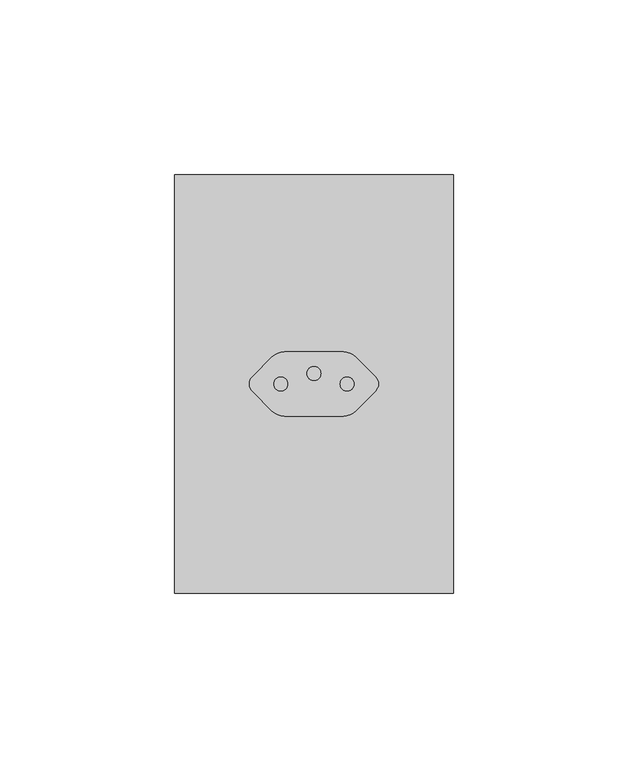
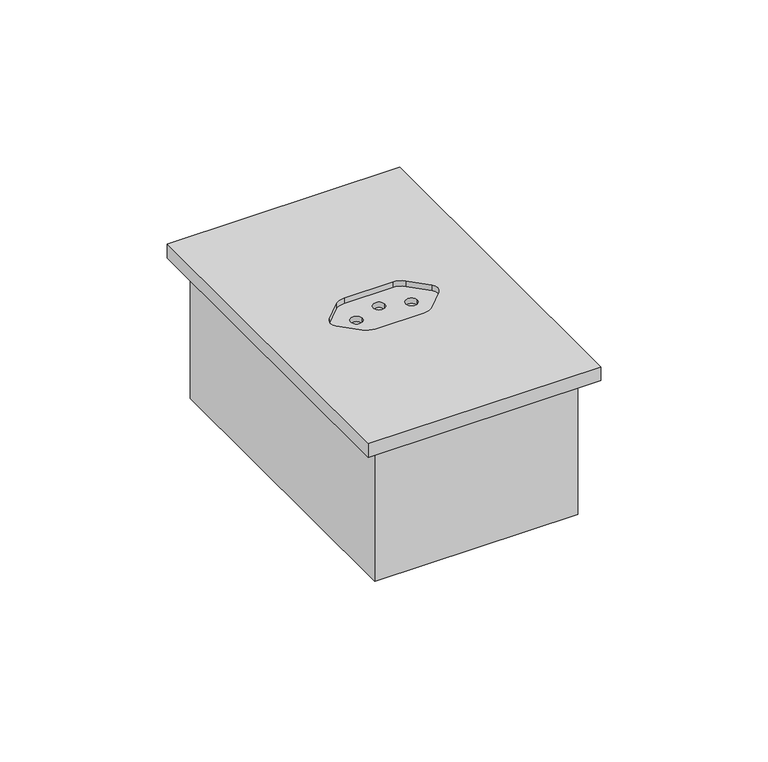
"""IFC4 building model written with IfcOpenShell, lengths in millimetres: proxy geometry, CAIXA VERTICE V7 : Tomada 10A 1s."""

from ifc_helpers import new_model, si_unit, frame, origin, place, context, project, spatial, polyline, circle_curve, faceted_brep, source, transform, mapped, element, save
from ifc_brep_helpers import plane_surface, revolved_surface, advanced_brep


def electrical_fixtures_2885af8d(model_context):
    return source(origin(), model_context, "Body", "SolidModel", [
        faceted_brep([(35.0, 455.0, 0.0), (-35.0, 455.0, 0.0), (-35.0, 345.0, 0.0), (35.0, 345.0, 0.0), (33.0, 453.0, 0.0), (33.0, 347.0, 0.0), (-33.0, 347.0, 0.0), (-33.0, 453.0, 0.0), (33.0, 347.0, -48.0), (33.0, 453.0, -48.0), (-33.0, 453.0, -48.0), (-33.0, 347.0, -48.0), (35.0, 455.0, -50.0), (35.0, 345.0, -50.0), (-35.0, 345.0, -50.0), (-35.0, 455.0, -50.0)], [[[0, 1, 2, 3], [4, 5, 6, 7]], [[8, 9, 10, 11]], [[12, 13, 14, 15]], [[12, 15, 1, 0]], [[1, 15, 14, 2]], [[2, 14, 13, 3]], [[3, 13, 12, 0]], [[5, 4, 9, 8]], [[6, 5, 8, 11]], [[7, 6, 11, 10]], [[4, 7, 10, 9]]]),
        advanced_brep(
        [(40.0, 460.0, 5.0), (-40.0, 460.0, 5.0), (-40.0, 340.0, 5.0), (40.0, 340.0, 5.0), (8.4215729, 390.75, 5.0), (-8.4215729, 390.75, 5.0), (-11.9571068, 392.2144661, 5.0), (-17.6213203, 397.8786797, 5.0), (-17.6213203, 402.1213203, 5.0), (-11.9571068, 407.7855339, 5.0), (-8.4215729, 409.25, 5.0), (8.4215729, 409.25, 5.0), (11.9571068, 407.7855339, 5.0), (17.6213203, 402.1213203, 5.0), (17.6213203, 397.8786797, 5.0), (11.9571068, 392.2144661, 5.0), (-40.0, 460.0, 0.0), (40.0, 460.0, 0.0), (40.0, 340.0, 0.0), (-40.0, 340.0, 0.0), (8.4215729, 390.75, 3.0), (11.9571068, 392.2144661, 3.0), (17.6213203, 397.8786797, 3.0), (17.6213203, 402.1213203, 3.0), (11.9571068, 407.7855339, 3.0), (8.4215729, 409.25, 3.0), (-8.4215729, 409.25, 3.0), (-11.9571068, 407.7855339, 3.0), (-17.6213203, 402.1213203, 3.0), (-17.6213203, 397.8786797, 3.0), (-11.9571068, 392.2144661, 3.0), (-8.4215729, 390.75, 3.0), (-7.5, 400.0, 3.0), (-11.5, 400.0, 3.0), (11.5, 400.0, 3.0), (7.5, 400.0, 3.0), (2.0, 403.0, 3.0), (-2.0, 403.0, 3.0), (-11.5, 400.0, 1.0), (-7.5, 400.0, 1.0), (7.5, 400.0, 1.0), (11.5, 400.0, 1.0), (-2.0, 403.0, 1.0), (2.0, 403.0, 1.0)],
        [
            (0, 1),
            (1, 2),
            (2, 3),
            (3, 0),
            (4, 5),
            (5, 6, circle_curve(frame((-8.4215729, 395.75, 5.0), z_axis=(0.0, 0.0, -1.0), x_axis=(-1.0, 0.0, 0.0)), 5.0)),
            (6, 7),
            (7, 8, circle_curve(frame((-15.5, 400.0, 5.0), z_axis=(0.0, 0.0, -1.0), x_axis=(-1.0, 0.0, 0.0)), 3.0)),
            (8, 9),
            (9, 10, circle_curve(frame((-8.4215729, 404.25, 5.0), z_axis=(0.0, 0.0, -1.0), x_axis=(-1.0, 0.0, 0.0)), 5.0)),
            (10, 11),
            (11, 12, circle_curve(frame((8.4215729, 404.25, 5.0), z_axis=(0.0, 0.0, -1.0), x_axis=(-1.0, 0.0, 0.0)), 5.0)),
            (12, 13),
            (13, 14, circle_curve(frame((15.5, 400.0, 5.0), z_axis=(0.0, 0.0, -1.0), x_axis=(-1.0, 0.0, 0.0)), 3.0)),
            (14, 15),
            (15, 4, circle_curve(frame((8.4215729, 395.75, 5.0), z_axis=(0.0, 0.0, -1.0), x_axis=(-1.0, 0.0, 0.0)), 5.0)),
            (16, 17),
            (17, 18),
            (18, 19),
            (19, 16),
            (0, 17),
            (16, 1),
            (19, 2),
            (18, 3),
            (20, 21, circle_curve(frame((8.4215729, 395.75, 3.0), z_axis=(0.0, 0.0, 1.0), x_axis=(-1.0, 0.0, 0.0)), 5.0)),
            (21, 22),
            (22, 23, circle_curve(frame((15.5, 400.0, 3.0), z_axis=(0.0, 0.0, 1.0), x_axis=(-1.0, 0.0, 0.0)), 3.0)),
            (23, 24),
            (24, 25, circle_curve(frame((8.4215729, 404.25, 3.0), z_axis=(0.0, 0.0, 1.0), x_axis=(-1.0, 0.0, 0.0)), 5.0)),
            (25, 26),
            (26, 27, circle_curve(frame((-8.4215729, 404.25, 3.0), z_axis=(0.0, 0.0, 1.0), x_axis=(-1.0, 0.0, 0.0)), 5.0)),
            (27, 28),
            (28, 29, circle_curve(frame((-15.5, 400.0, 3.0), z_axis=(0.0, 0.0, 1.0), x_axis=(-1.0, 0.0, 0.0)), 3.0)),
            (29, 30),
            (30, 31, circle_curve(frame((-8.4215729, 395.75, 3.0), z_axis=(0.0, 0.0, 1.0), x_axis=(-1.0, 0.0, 0.0)), 5.0)),
            (31, 20),
            (32, 33, circle_curve(frame((-9.5, 400.0, 3.0), z_axis=(0.0, 0.0, -1.0), x_axis=(1.0, 2.301812013077709e-12, 0.0)), 2.0)),
            (33, 32, circle_curve(frame((-9.5, 400.0, 3.0), z_axis=(0.0, 0.0, -1.0), x_axis=(1.0, 2.301812013077709e-12, 0.0)), 2.0)),
            (34, 35, circle_curve(frame((9.5, 400.0, 3.0), z_axis=(0.0, 0.0, -1.0), x_axis=(1.0, 2.301812013077709e-12, 0.0)), 2.0)),
            (35, 34, circle_curve(frame((9.5, 400.0, 3.0), z_axis=(0.0, 0.0, -1.0), x_axis=(1.0, 2.301812013077709e-12, 0.0)), 2.0)),
            (36, 37, circle_curve(frame((0.0, 403.0, 3.0), z_axis=(0.0, 0.0, -1.0), x_axis=(1.0, 2.301812013077709e-12, 0.0)), 2.0)),
            (37, 36, circle_curve(frame((0.0, 403.0, 3.0), z_axis=(0.0, 0.0, -1.0), x_axis=(1.0, 2.301812013077709e-12, 0.0)), 2.0)),
            (31, 5),
            (4, 20),
            (30, 6),
            (29, 7),
            (28, 8),
            (27, 9),
            (26, 10),
            (25, 11),
            (24, 12),
            (23, 13),
            (22, 14),
            (21, 15),
            (38, 39, circle_curve(frame((-9.5, 400.0, 1.0), z_axis=(0.0, 0.0, 1.0), x_axis=(1.0, 2.301812013077709e-12, 0.0)), 2.0)),
            (39, 38, circle_curve(frame((-9.5, 400.0, 1.0), z_axis=(0.0, 0.0, 1.0), x_axis=(1.0, 2.301812013077709e-12, 0.0)), 2.0)),
            (40, 41, circle_curve(frame((9.5, 400.0, 1.0), z_axis=(0.0, 0.0, 1.0), x_axis=(1.0, 2.301812013077709e-12, 0.0)), 2.0)),
            (41, 40, circle_curve(frame((9.5, 400.0, 1.0), z_axis=(0.0, 0.0, 1.0), x_axis=(1.0, 2.301812013077709e-12, 0.0)), 2.0)),
            (42, 43, circle_curve(frame((0.0, 403.0, 1.0), z_axis=(0.0, 0.0, 1.0), x_axis=(1.0, 2.301812013077709e-12, 0.0)), 2.0)),
            (43, 42, circle_curve(frame((0.0, 403.0, 1.0), z_axis=(0.0, 0.0, 1.0), x_axis=(1.0, 2.301812013077709e-12, 0.0)), 2.0)),
            (32, 39),
            (38, 33),
            (34, 41),
            (40, 35),
            (36, 43),
            (42, 37),
        ],
        [
            plane_surface(frame((-60.0, 460.0, 5.0), z_axis=(0.0, 0.0, 1.0), x_axis=(-1.0, 0.0, 0.0))),
            plane_surface(frame((-60.0, 460.0, 0.0), z_axis=(0.0, 0.0, -1.0), x_axis=(1.0, 0.0, 0.0))),
            plane_surface(frame((40.0, 460.0, 5.0), z_axis=(0.0, 1.0, 0.0), x_axis=(0.0, 0.0, -1.0))),
            plane_surface(frame((-40.0, 460.0, 5.0), z_axis=(-1.0, 0.0, 0.0), x_axis=(0.0, 0.0, -1.0))),
            plane_surface(frame((-40.0, 340.0, 5.0), z_axis=(0.0, -1.0, 0.0), x_axis=(0.0, 0.0, -1.0))),
            plane_surface(frame((40.0, 340.0, 5.0), z_axis=(1.0, 0.0, 0.0), x_axis=(0.0, 0.0, -1.0))),
            plane_surface(frame((3.4215729, 395.75, 3.0), z_axis=(0.0, 0.0, 1.0), x_axis=(0.0, 1.0, 0.0))),
            plane_surface(frame((-8.4215729, 390.75, 5.0), z_axis=(0.0, 1.0, 0.0), x_axis=(0.0, 0.0, -1.0))),
            revolved_surface(polyline([(-13.4215729, 395.75, 5.0), (-13.4215729, 395.75, 3.0)]), (-8.4215729, 395.75, 3.0), (0.0, 0.0, 1.0)),
            plane_surface(frame((-17.6213203, 397.8786797, 5.0), z_axis=(0.7071067811865045, 0.7071067811865905, 0.0), x_axis=(0.0, 0.0, -1.0))),
            revolved_surface(polyline([(-18.5, 400.0, 5.0), (-18.5, 400.0, 3.0)]), (-15.5, 400.0, 3.0), (0.0, 0.0, 1.0)),
            plane_surface(frame((-11.9571068, 407.7855339, 5.0), z_axis=(0.7071067811865515, -0.7071067811865437, 0.0), x_axis=(0.0, 0.0, -1.0))),
            revolved_surface(polyline([(-13.4215729, 404.25, 5.0), (-13.4215729, 404.25, 3.0)]), (-8.4215729, 404.25, 3.0), (0.0, 0.0, 1.0)),
            plane_surface(frame((8.4215729, 409.25, 5.0), z_axis=(0.0, -1.0, 0.0), x_axis=(0.0, 0.0, -1.0))),
            revolved_surface(polyline([(3.4215728999999993, 404.25, 5.0), (3.4215728999999993, 404.25, 3.0)]), (8.4215729, 404.25, 3.0), (0.0, 0.0, 1.0)),
            plane_surface(frame((17.6213203, 402.1213203, 5.0), z_axis=(-0.7071067811865307, -0.7071067811865643, 0.0), x_axis=(0.0, 0.0, -1.0))),
            revolved_surface(polyline([(12.5, 400.0, 5.0), (12.5, 400.0, 3.0)]), (15.5, 400.0, 3.0), (0.0, 0.0, 1.0)),
            plane_surface(frame((11.9571068, 392.2144661, 5.0), z_axis=(-0.7071067811865893, 0.7071067811865058, 0.0), x_axis=(0.0, 0.0, -1.0))),
            revolved_surface(polyline([(3.4215728999999993, 395.75, 5.0), (3.4215728999999993, 395.75, 3.0)]), (8.4215729, 395.75, 3.0), (0.0, 0.0, 1.0)),
            plane_surface(frame((-7.5, 400.0, 1.0), z_axis=(0.0, 0.0, 1.0), x_axis=(2.301812013077709e-12, -1.0, 0.0))),
            revolved_surface(polyline([(-7.5, 400.0000000000046, 3.0), (-7.5, 400.0000000000046, 1.0)]), (-9.5, 400.0, 1.0), (0.0, 0.0, 1.0)),
            revolved_surface(polyline([(11.5, 400.0000000000046, 3.0), (11.5, 400.0000000000046, 1.0)]), (9.5, 400.0, 5.0), (0.0, 0.0, 1.0)),
            revolved_surface(polyline([(2.0, 403.0000000000046, 3.0), (2.0, 403.0000000000046, 1.0)]), (0.0, 403.0, 5.0), (0.0, 0.0, 1.0)),
        ],
        [
            (0, [[1, 2, 3, 4], [5, 6, 7, 8, 9, 10, 11, 12, 13, 14, 15, 16]]),
            (1, [[17, 18, 19, 20]]),
            (2, [[-1, 21, -17, 22]]),
            (3, [[-2, -22, -20, 23]]),
            (4, [[-3, -23, -19, 24]]),
            (5, [[-4, -24, -18, -21]]),
            (6, [[25, 26, 27, 28, 29, 30, 31, 32, 33, 34, 35, 36], [37, 38], [39, 40], [41, 42]]),
            (7, [[-36, 43, -5, 44]]),
            (8, [[-35, 45, -6, -43]]),
            (9, [[-34, 46, -7, -45]]),
            (10, [[-33, 47, -8, -46]]),
            (11, [[-32, 48, -9, -47]]),
            (12, [[-31, 49, -10, -48]]),
            (13, [[-30, 50, -11, -49]]),
            (14, [[-29, 51, -12, -50]]),
            (15, [[-28, 52, -13, -51]]),
            (16, [[-27, 53, -14, -52]]),
            (17, [[-26, 54, -15, -53]]),
            (18, [[-25, -44, -16, -54]]),
            (19, [[55, 56]]),
            (19, [[57, 58]]),
            (19, [[59, 60]]),
            (20, [[-37, 61, -55, 62]]),
            (20, [[-38, -62, -56, -61]]),
            (21, [[-39, 63, -57, 64]]),
            (21, [[-40, -64, -58, -63]]),
            (22, [[-41, 65, -59, 66]]),
            (22, [[-42, -66, -60, -65]]),
        ],
    ),
    ])


if __name__ == "__main__":
    model = new_model("IFC4")
    model_context = context("Model", 3, world=origin())
    ifc_project = project(units=[si_unit("LENGTHUNIT", "METRE", prefix="MILLI")], contexts=[model_context])
    site = spatial("IfcSite", under=ifc_project)
    building = spatial("IfcBuilding", under=site)
    placement = place(None, origin())
    electrical_fixtures_shape = electrical_fixtures_2885af8d(model_context)
    element("IfcBuildingElementProxy", 1, Name="CAIXA VERTICE V7 : Tomada 10A 1s", ObjectType="CAIXA VERTICE V7 : Tomada 10A 1s", at=placement, inside=building, context=model_context, shape_type="MappedRepresentation", body=[
        mapped(electrical_fixtures_shape, transform((0.0, 0.0, 0.0), x_axis=(1.0, 0.0, 0.0), y_axis=(0.0, 1.0, 0.0), z_axis=(0.0, 0.0, 1.0))),
    ])
    save(model, "model.ifc")

# Revit data of these elements
# Type "CAIXA VERTICE V7 : Tomada 10A 1s"
#   URL = "www.facebook.com/verticetreinamentos"
#   SEÇÃO [instance default] = ""
#   Rotação [instance default] = 0.00°
#   LARGURA DA TAMPA = 0.08 m
#   BORDA = 0.01 m
#   ALTURA DE INSTALAÇÃO [instance default] = 1.10 m
#   Distância Anotação [instance default] = 0.0015 m
#   ALTURA DA TAMPA = 0.12 m
#   Vertical [instance default] = yes
#   VER SEÇÃO [instance default] = no
#   SHADE ESQ [instance default] = no
#   SHADE DIR [instance default] = yes
#   HORIZONTAL [instance default] = no
#   ANDAR COM A LEGENDA [instance default] = 0
#   Material Tampa [instance default] = Plástico, branco opaco
#   Caixa = element 1798514
#   Anotação = element 1798528
#   Default Elevation = 0
# Element 1 (IfcBuildingElementProxy, "CAIXA VERTICE V7 : Tomada 10A 1s")
#   ALTURA DE INSTALAÇÃO = 0.40 m
#   VER SEÇÃO = yes
#   SHADE DIR = no
#   Materials on its faces: "Plástico, branco opaco"
# Materials
#   "Plástico, branco opaco": class "Plástico", colour RGB 120 120 120, transparency 0, Description = "Plastic, generic, opaque white", Cost = 0
